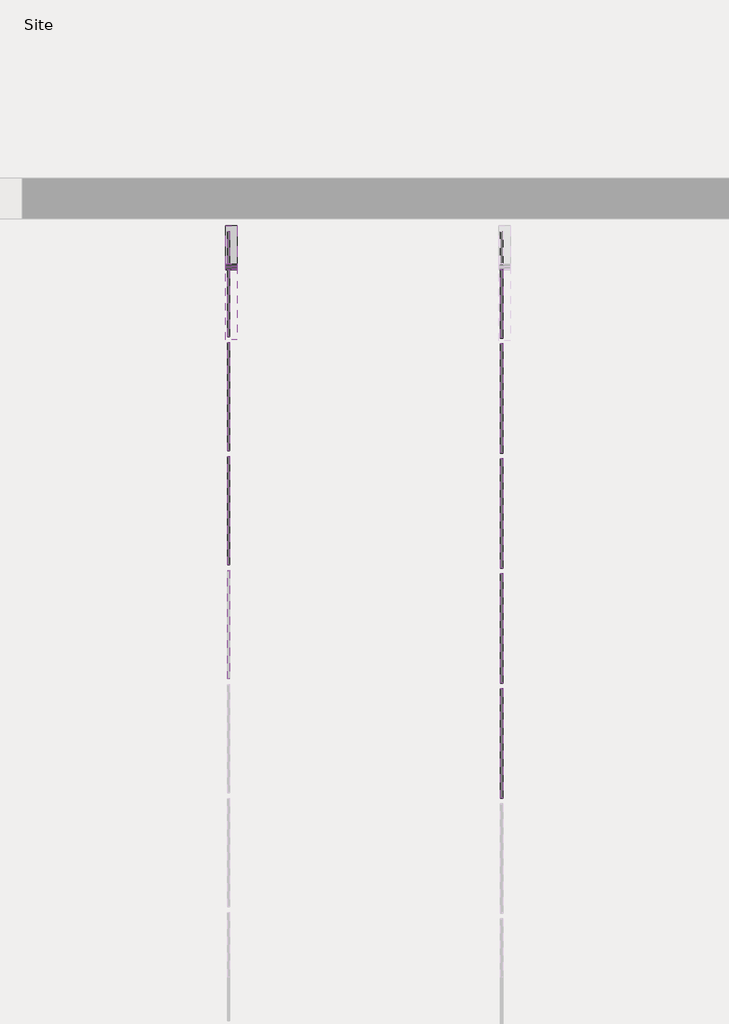
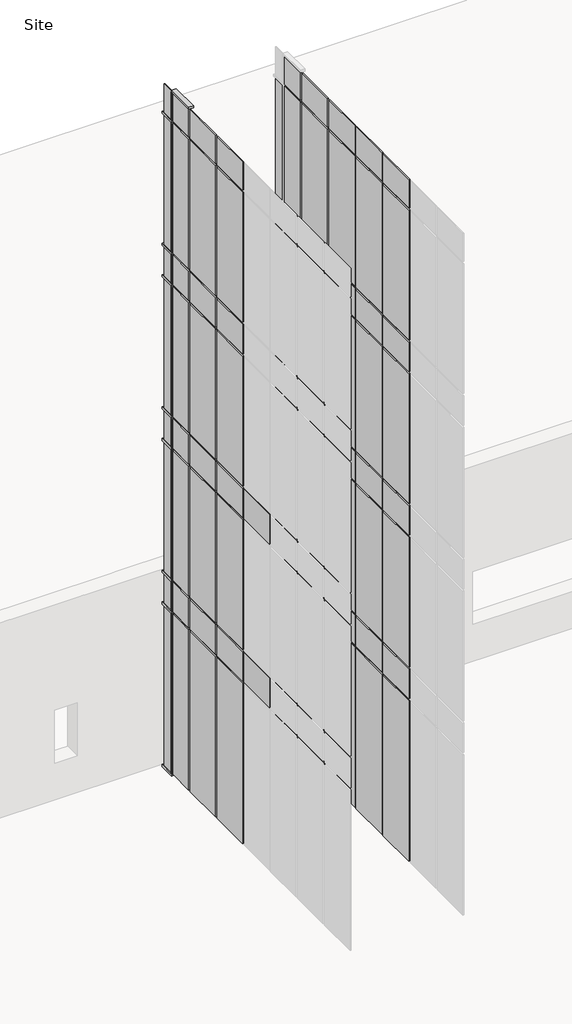
# One storey, part 3 of 4: 81 plates, 17 members.
"""IFC4 building model written with IfcOpenShell, lengths in millimetres."""

import ifcopenshell
import ifcopenshell.guid

model = None  # the IFC model being written
_history = None  # IfcOwnerHistory: only IFC2X3 demands one
_inside = {}  # id of a spatial element -> (the spatial element, [elements in it])
_under = {}  # id of a project, library or spatial element -> (it, [spatial elements below it])
_declared = {}  # id of a project -> (the project, [libraries it declares])
_typed = {}  # id of a type object -> (the type object, [elements of that type])
_made_of = {}  # id of a material, layer set ... -> (it, [elements and type objects made of it])


def new_model(schema):
    """Start an empty IFC model of exactly this schema.

    Asked for "IFC4X3", IfcOpenShell would pick the latest addendum, in which some entities
    have other attributes; the version numbers below select the first issue.
    IFC2X3 requires an IfcOwnerHistory on every rooted entity: one is made here for all.
    """
    global model, _history
    if schema == "IFC4X3":
        model = ifcopenshell.file(schema_version=(4, 3, 0, 0))
    else:
        model = ifcopenshell.file(schema=schema)
    _inside.clear()
    _under.clear()
    _declared.clear()
    _typed.clear()
    _made_of.clear()
    _history = None
    if model.schema == "IFC2X3":
        org = make("IfcOrganization", Name="unknown")
        user = make(
            "IfcPersonAndOrganization",
            ThePerson=make("IfcPerson", FamilyName="unknown"),
            TheOrganization=org,
        )
        app = make(
            "IfcApplication",
            ApplicationDeveloper=org,
            Version="unknown",
            ApplicationFullName="unknown",
            ApplicationIdentifier="unknown",
        )
        _history = make(
            "IfcOwnerHistory",
            OwningUser=user,
            OwningApplication=app,
            ChangeAction="ADDED",
            CreationDate=0,
        )
    return model


def make(cls, **values):
    """One entity of the class cls with the attributes given. An attribute that is None is left unset."""
    return model.create_entity(
        cls, **{name: value for name, value in values.items() if value is not None}
    )


def rooted(cls, **values):
    """An entity with a GlobalId (a new one), such as an element, a storey or a relation."""
    return make(cls, GlobalId=ifcopenshell.guid.new(), OwnerHistory=_history, **values)


def si_unit(unit_type, name, prefix=None):
    """IfcSIUnit, for example si_unit("LENGTHUNIT", "METRE", prefix="MILLI")."""
    return make("IfcSIUnit", UnitType=unit_type, Prefix=prefix, Name=name)


def assignment(units):
    """IfcUnitAssignment: the units of a project."""
    return None if units is None else make("IfcUnitAssignment", Units=units)


def point(xyz):
    """IfcCartesianPoint."""
    return None if xyz is None else make("IfcCartesianPoint", Coordinates=xyz)


def direction(xyz):
    """IfcDirection."""
    return None if xyz is None else make("IfcDirection", DirectionRatios=xyz)


def frame(location, z_axis=None, x_axis=None):
    """IfcAxis2Placement3D, a coordinate frame: its origin and axes. An axis left out is left unset."""
    return make(
        "IfcAxis2Placement3D",
        Location=point(location),
        Axis=direction(z_axis),
        RefDirection=direction(x_axis),
    )


def origin():
    """The frame at (0, 0, 0) with its axes left unset."""
    return frame((0.0, 0.0, 0.0))


def origin_with_axes():
    """The frame at (0, 0, 0) with the z axis (0, 0, 1) and the x axis (1, 0, 0) written out."""
    return frame((0.0, 0.0, 0.0), z_axis=(0.0, 0.0, 1.0), x_axis=(1.0, 0.0, 0.0))


def place(relative_to, where):
    """IfcLocalPlacement: puts the frame where relative to a parent placement (None: the world)."""
    return make(
        "IfcLocalPlacement", PlacementRelTo=relative_to, RelativePlacement=where
    )


def context(
    kind, dimensions, precision=None, world=None, true_north=None, identifier=None
):
    """IfcGeometricRepresentationContext, for example the 3D "Model" context."""
    return make(
        "IfcGeometricRepresentationContext",
        ContextIdentifier=identifier,
        ContextType=kind,
        CoordinateSpaceDimension=dimensions,
        Precision=precision,
        WorldCoordinateSystem=world,
        TrueNorth=true_north,
    )


def project(units=None, contexts=None):
    """IfcProject with its units and contexts."""
    return rooted(
        "IfcProject",
        Name="project",
        RepresentationContexts=contexts,
        UnitsInContext=assignment(units),
    )


def spatial(cls, under=None, at=None, **own):
    """A site, building, storey or space (cls), placed at a placement, below another one or the project."""
    s = rooted(cls, ObjectPlacement=at, **own)
    if under is not None:
        _under.setdefault(under.id(), (under, []))[1].append(s)
    return s


def polyline(points):
    """IfcPolyline through the points."""
    return make("IfcPolyline", Points=[point(p) for p in points])


def outline(outer, holes=None, kind="AREA"):
    """IfcArbitraryClosedProfileDef: a profile drawn as a closed curve; with holes, ...WithVoids."""
    if holes is None:
        return make("IfcArbitraryClosedProfileDef", ProfileType=kind, OuterCurve=outer)
    return make(
        "IfcArbitraryProfileDefWithVoids",
        ProfileType=kind,
        OuterCurve=outer,
        InnerCurves=holes,
    )


def extrude(swept, where, along, depth):
    """IfcExtrudedAreaSolid: the profile swept, set in the frame where, extruded along a direction by depth."""
    return make(
        "IfcExtrudedAreaSolid",
        SweptArea=swept,
        Position=where,
        ExtrudedDirection=direction(along),
        Depth=depth,
    )


def shape(context_of_items, identifier, shape_type, items):
    """IfcShapeRepresentation: the items that make up one representation, for example the "Body"."""
    return make(
        "IfcShapeRepresentation",
        ContextOfItems=context_of_items,
        RepresentationIdentifier=identifier,
        RepresentationType=shape_type,
        Items=items,
    )


def source(mapping_origin, context_of_items, identifier, shape_type, items):
    """IfcRepresentationMap: a shape defined once, which mapped items show again and again."""
    return make(
        "IfcRepresentationMap",
        MappingOrigin=mapping_origin,
        MappedRepresentation=shape(context_of_items, identifier, shape_type, items),
    )


def transform(
    local_origin,
    x_axis=None,
    y_axis=None,
    z_axis=None,
    scale=None,
    scale2=None,
    scale3=None,
    uniform=True,
):
    """IfcCartesianTransformationOperator3D, or its non-uniform kind. x_axis, y_axis, z_axis: its Axis1, 2, 3."""
    if uniform:
        return make(
            "IfcCartesianTransformationOperator3D",
            Axis1=direction(x_axis),
            Axis2=direction(y_axis),
            LocalOrigin=point(local_origin),
            Scale=scale,
            Axis3=direction(z_axis),
        )
    return make(
        "IfcCartesianTransformationOperator3DnonUniform",
        Axis1=direction(x_axis),
        Axis2=direction(y_axis),
        LocalOrigin=point(local_origin),
        Scale=scale,
        Axis3=direction(z_axis),
        Scale2=scale2,
        Scale3=scale3,
    )


def mapped(mapping_source, mapping_target):
    """IfcMappedItem: shows the shape of a source again, moved by a transform."""
    return make(
        "IfcMappedItem", MappingSource=mapping_source, MappingTarget=mapping_target
    )


def made_of(thing, what):
    """Note that an element or type object is made of a material, layer set ...; save() writes the relation."""
    if what is not None:
        _made_of.setdefault(what.id(), (what, []))[1].append(thing)
    return thing


def element(
    cls,
    number,
    at=None,
    inside=None,
    cuts=None,
    type_object=None,
    material=None,
    context=None,
    identifier="Body",
    shape_type=None,
    held_by="IfcProductDefinitionShape",
    body=None,
    shapes=None,
    **own,
):
    """One element of the class cls, such as IfcWall. Its Tag is "e" and its number.

    at: its placement. inside: the storey or other place that contains it. cuts: it is an
    opening in that element (IfcRelVoidsElement). A single representation is given by context,
    identifier, shape_type and body (its items); several are given by shapes. held_by: the class
    of the entity that holds the representations. save() writes the other relations.
    """
    e = rooted(cls, Tag="e%d" % number, ObjectPlacement=at, **own)
    if body is not None:
        shapes = [shape(context, identifier, shape_type, body)]
    if shapes is not None:
        e.Representation = make(held_by, Representations=shapes)
    if inside is not None:
        _inside.setdefault(inside.id(), (inside, []))[1].append(e)
    if cuts is not None:
        rooted(
            "IfcRelVoidsElement", RelatingBuildingElement=cuts, RelatedOpeningElement=e
        )
    if type_object is not None:
        _typed.setdefault(type_object.id(), (type_object, []))[1].append(e)
    return made_of(e, material)


def aggregate(whole, parts):
    """IfcRelAggregates: a whole, such as a stair, and the parts it consists of."""
    return rooted("IfcRelAggregates", RelatingObject=whole, RelatedObjects=parts)


def save(model, path):
    """Write the relations noted so far, then the file.

    IfcRelAggregates (storeys below a building ...), IfcRelContainedInSpatialStructure (elements
    in a storey), IfcRelDefinesByType, IfcRelAssociatesMaterial and IfcRelDeclares: one each for
    every whole, place, type object, material and project.
    """
    for whole, parts in _under.values():
        aggregate(whole, parts)
    for where, things in _inside.values():
        rooted(
            "IfcRelContainedInSpatialStructure",
            RelatedElements=things,
            RelatingStructure=where,
        )
    for kind, things in _typed.values():
        rooted("IfcRelDefinesByType", RelatedObjects=things, RelatingType=kind)
    for what, things in _made_of.values():
        rooted("IfcRelAssociatesMaterial", RelatedObjects=things, RelatingMaterial=what)
    for by, libraries in _declared.values():
        rooted("IfcRelDeclares", RelatingContext=by, RelatedDefinitions=libraries)
    model.write(path)


def member_5d07894b(model_context):
    return source(origin(), model_context, "Body", "SweptSolid", [
        extrude(outline(polyline([(31.75, 63.5), (31.75, -63.5), (-31.75, -63.5), (-31.75, 63.5), (31.75, 63.5)])), frame((0.0, 0.0, -4629.15), z_axis=(0.0, 0.0, 1.0), x_axis=(1.0, 0.0, 0.0)), (0.0, 0.0, 1.0), 4629.15),
    ])


def member_3ba9e939(model_context):
    return source(origin(), model_context, "Body", "SweptSolid", [
        extrude(outline(polyline([(31.75, 63.5), (31.75, -63.5), (-31.75, -63.5), (-31.75, 63.5), (31.75, 63.5)])), frame((0.0, 0.0, -3746.5), z_axis=(0.0, 0.0, 1.0), x_axis=(1.0, 0.0, 0.0)), (0.0, 0.0, 1.0), 3746.5),
    ])


def member_ad567e07(model_context):
    return source(origin(), model_context, "Body", "SweptSolid", [
        extrude(outline(polyline([(31.75, 63.5), (31.75, -63.5), (-31.75, -63.5), (-31.75, 63.5), (31.75, 63.5)])), frame((0.0, 0.0, -819.15), z_axis=(0.0, 0.0, 1.0), x_axis=(1.0, 0.0, 0.0)), (0.0, 0.0, 1.0), 819.15),
    ])


def member_7db1855a(model_context):
    return source(origin(), model_context, "Body", "SweptSolid", [
        extrude(outline(polyline([(31.75, 63.5), (31.75, -63.5), (-31.75, -63.5), (-31.75, 63.5), (31.75, 63.5)])), frame((0.0, 0.0, -850.9), z_axis=(0.0, 0.0, 1.0), x_axis=(1.0, 0.0, 0.0)), (0.0, 0.0, 1.0), 850.9),
    ])


def member_7227ddca(model_context):
    return source(origin(), model_context, "Body", "SweptSolid", [
        extrude(outline(polyline([(0.0, 63.5), (0.0, -63.5), (-63.5, -63.5), (-63.5, 63.5), (0.0, 63.5)])), frame((0.0, 0.0, -813.7989637), z_axis=(0.0, 0.0, 1.0), x_axis=(1.0, 0.0, 0.0)), (0.0, 0.0, 1.0), 813.7989637),
    ])


def member_ffd4c858(model_context):
    return source(origin(), model_context, "Body", "SweptSolid", [
        extrude(outline(polyline([(31.75, 63.5), (31.75, -63.5), (-31.75, -63.5), (-31.75, 63.5), (31.75, 63.5)])), frame((0.0, 0.0, -457.2), z_axis=(0.0, 0.0, 1.0), x_axis=(1.0, 0.0, 0.0)), (0.0, 0.0, 1.0), 457.2),
    ])


def member_15823cb3(model_context):
    return source(origin(), model_context, "Body", "SweptSolid", [
        extrude(outline(polyline([(0.0, 63.5), (0.0, -63.5), (-63.5, -63.5), (-63.5, 63.5), (0.0, 63.5)])), frame((0.0, 0.0, -457.2), z_axis=(0.0, 0.0, 1.0), x_axis=(1.0, 0.0, 0.0)), (0.0, 0.0, 1.0), 457.2),
    ])


def system_panel_glazed_26f8e022(model_context):
    return source(origin(), model_context, "Body", "SweptSolid", [
        extrude(outline(polyline([(603.7494819, 19.05), (-603.7494819, 19.05), (-603.7494819, 44.45), (603.7494819, 44.45), (603.7494819, 19.05)])), origin_with_axes(), (0.0, 0.0, 1.0), 4629.15),
    ])


def system_panel_glazed_31d10065(model_context):
    return source(origin(), model_context, "Body", "SweptSolid", [
        extrude(outline(polyline([(609.6, 19.05), (-609.6, 19.05), (-609.6, 44.45), (609.6, 44.45), (609.6, 19.05)])), origin_with_axes(), (0.0, 0.0, 1.0), 4629.15),
    ])


def system_panel_glazed_ccbaed92(model_context):
    return source(origin(), model_context, "Body", "SweptSolid", [
        extrude(outline(polyline([(375.1494819, 19.05), (-375.1494819, 19.05), (-375.1494819, 44.45), (375.1494819, 44.45), (375.1494819, 19.05)])), origin_with_axes(), (0.0, 0.0, 1.0), 4629.15),
    ])


def system_panel_glazed_7dca4fa5(model_context):
    return source(origin(), model_context, "Body", "SweptSolid", [
        extrude(outline(polyline([(381.0, 19.05), (-381.0, 19.05), (-381.0, 44.45), (381.0, 44.45), (381.0, 19.05)])), origin_with_axes(), (0.0, 0.0, 1.0), 4629.15),
    ])


def system_panel_glazed_2b3d2baa(model_context):
    return source(origin(), model_context, "Body", "SweptSolid", [
        extrude(outline(polyline([(609.6, 19.05), (-609.6, 19.05), (-609.6, 44.45), (609.6, 44.45), (609.6, 19.05)])), origin_with_axes(), (0.0, 0.0, 1.0), 3746.5),
    ])


def system_panel_glazed_7e289b92(model_context):
    return source(origin(), model_context, "Body", "SweptSolid", [
        extrude(outline(polyline([(381.0, 19.05), (-381.0, 19.05), (-381.0, 44.45), (381.0, 44.45), (381.0, 19.05)])), origin_with_axes(), (0.0, 0.0, 1.0), 3746.5),
    ])


def system_panel_glazed_8fe7ab7d(model_context):
    return source(origin(), model_context, "Body", "SweptSolid", [
        extrude(outline(polyline([(609.6, 19.05), (-609.6, 19.05), (-609.6, 44.45), (609.6, 44.45), (609.6, 19.05)])), origin_with_axes(), (0.0, 0.0, 1.0), 850.9),
    ])


def system_panel_glazed_4fa5cbd7(model_context):
    return source(origin(), model_context, "Body", "SweptSolid", [
        extrude(outline(polyline([(381.0, 19.05), (-381.0, 19.05), (-381.0, 44.45), (381.0, 44.45), (381.0, 19.05)])), origin_with_axes(), (0.0, 0.0, 1.0), 850.9),
    ])


def system_panel_glazed_636dec6d(model_context):
    return source(origin(), model_context, "Body", "SweptSolid", [
        extrude(outline(polyline([(609.6, 19.05), (-609.6, 19.05), (-609.6, 44.45), (609.6, 44.45), (609.6, 19.05)])), origin_with_axes(), (0.0, 0.0, 1.0), 819.15),
    ])


def system_panel_glazed_99ba6c15(model_context):
    return source(origin(), model_context, "Body", "SweptSolid", [
        extrude(outline(polyline([(381.0, 19.05), (-381.0, 19.05), (-381.0, 44.45), (381.0, 44.45), (381.0, 19.05)])), origin_with_axes(), (0.0, 0.0, 1.0), 819.15),
    ])


def system_panel_glazed_35bb093a(model_context):
    return source(origin(), model_context, "Body", "SweptSolid", [
        extrude(outline(polyline([(603.7494819, 19.05), (-603.7494819, 19.05), (-603.7494819, 44.45), (603.7494819, 44.45), (603.7494819, 19.05)])), origin_with_axes(), (0.0, 0.0, 1.0), 3746.5),
    ])


def system_panel_glazed_f4d1d7f7(model_context):
    return source(origin(), model_context, "Body", "SweptSolid", [
        extrude(outline(polyline([(375.1494819, 19.05), (-375.1494819, 19.05), (-375.1494819, 44.45), (375.1494819, 44.45), (375.1494819, 19.05)])), origin_with_axes(), (0.0, 0.0, 1.0), 3746.5),
    ])


def system_panel_glazed_6e853645(model_context):
    return source(origin(), model_context, "Body", "SweptSolid", [
        extrude(outline(polyline([(180.975, 19.05), (-180.975, 19.05), (-180.975, 44.45), (180.975, 44.45), (180.975, 19.05)])), origin_with_axes(), (0.0, 0.0, 1.0), 4629.15),
    ])


def system_panel_glazed_5cc7900c(model_context):
    return source(origin(), model_context, "Body", "SweptSolid", [
        extrude(outline(polyline([(180.975, 19.05), (-180.975, 19.05), (-180.975, 44.45), (180.975, 44.45), (180.975, 19.05)])), origin_with_axes(), (0.0, 0.0, 1.0), 850.9),
    ])


def system_panel_glazed_032e4dab(model_context):
    return source(origin(), model_context, "Body", "SweptSolid", [
        extrude(outline(polyline([(180.975, 19.05), (-180.975, 19.05), (-180.975, 44.45), (180.975, 44.45), (180.975, 19.05)])), origin_with_axes(), (0.0, 0.0, 1.0), 3746.5),
    ])


def system_panel_metal_panel_947f48db(model_context):
    return source(origin(), model_context, "Body", "SweptSolid", [
        extrude(outline(polyline([(603.7494819, 19.05), (-603.7494819, 19.05), (-603.7494819, 44.45), (603.7494819, 44.45), (603.7494819, 19.05)])), origin_with_axes(), (0.0, 0.0, 1.0), 819.15),
    ])


def system_panel_metal_panel_e2dbf0ce(model_context):
    return source(origin(), model_context, "Body", "SweptSolid", [
        extrude(outline(polyline([(375.1494819, 19.05), (-375.1494819, 19.05), (-375.1494819, 44.45), (375.1494819, 44.45), (375.1494819, 19.05)])), origin_with_axes(), (0.0, 0.0, 1.0), 819.15),
    ])


def system_panel_metal_panel_dcd9a435(model_context):
    return source(origin(), model_context, "Body", "SweptSolid", [
        extrude(outline(polyline([(603.7494819, 19.05), (-603.7494819, 19.05), (-603.7494819, 44.45), (603.7494819, 44.45), (603.7494819, 19.05)])), origin_with_axes(), (0.0, 0.0, 1.0), 850.9),
    ])


def system_panel_metal_panel_ab4ce9b6(model_context):
    return source(origin(), model_context, "Body", "SweptSolid", [
        extrude(outline(polyline([(375.1494819, 19.05), (-375.1494819, 19.05), (-375.1494819, 44.45), (375.1494819, 44.45), (375.1494819, 19.05)])), origin_with_axes(), (0.0, 0.0, 1.0), 850.9),
    ])


def system_panel_glazed_cc98a0ec(model_context):
    return source(origin(), model_context, "Body", "SweptSolid", [
        extrude(outline(polyline([(180.975, 19.05), (-180.975, 19.05), (-180.975, 44.45), (180.975, 44.45), (180.975, 19.05)])), origin_with_axes(), (0.0, 0.0, 1.0), 819.15),
    ])


model = new_model("IFC4")

# Units and contexts
model_context = context("Model", 3, world=origin())
ifc_project = project(units=[si_unit("LENGTHUNIT", "METRE", prefix="MILLI")], contexts=[model_context])

# Site, building, storey
site = spatial("IfcSite", under=ifc_project)
building = spatial("IfcBuilding", under=site)
storey = spatial("IfcBuildingStorey", under=building, Name="Site", Elevation=-152.4)

# Members
placement = place(None, origin())
member_shape = member_5d07894b(model_context)
element("IfcMember", 1, ObjectType="Rectangular Mullion1 : 2.5\" x 5\" rectangular", at=placement, inside=storey, context=model_context, shape_type="MappedRepresentation", body=[
    mapped(member_shape, transform((7830.8276119, 37629.311889, -88.9), x_axis=(0.0, 1.0, 0.0), y_axis=(1.0, 0.0, 0.0), z_axis=(0.0, 0.0, -1.0))),
])
member_2_shape = member_3ba9e939(model_context)
element("IfcMember", 2, ObjectType="Rectangular Mullion1 : 2.5\" x 5\" rectangular", at=placement, inside=storey, context=model_context, shape_type="MappedRepresentation", body=[
    mapped(member_2_shape, transform((7830.8276119, 37629.311889, 14966.95), x_axis=(0.0, 1.0, 0.0), y_axis=(1.0, 0.0, 0.0), z_axis=(0.0, 0.0, -1.0))),
])
element("IfcMember", 3, ObjectType="Rectangular Mullion1 : 2.5\" x 5\" rectangular", at=placement, inside=storey, context=model_context, shape_type="MappedRepresentation", body=[
    mapped(member_2_shape, transform((7830.8276119, 37629.311889, 10242.55), x_axis=(0.0, 1.0, 0.0), y_axis=(1.0, 0.0, 0.0), z_axis=(0.0, 0.0, -1.0))),
])
element("IfcMember", 4, ObjectType="Rectangular Mullion1 : 2.5\" x 5\" rectangular", at=placement, inside=storey, context=model_context, shape_type="MappedRepresentation", body=[
    mapped(member_2_shape, transform((7830.8276119, 37629.311889, 5518.15), x_axis=(0.0, 1.0, 0.0), y_axis=(1.0, 0.0, 0.0), z_axis=(0.0, 0.0, -1.0))),
])
member_3_shape = member_ad567e07(model_context)
element("IfcMember", 5, ObjectType="Rectangular Mullion1 : 2.5\" x 5\" rectangular", at=placement, inside=storey, context=model_context, shape_type="MappedRepresentation", body=[
    mapped(member_3_shape, transform((7830.8276119, 37629.311889, 18776.95), x_axis=(0.0, 1.0, 0.0), y_axis=(1.0, 0.0, 0.0), z_axis=(0.0, 0.0, -1.0))),
])
member_4_shape = member_7db1855a(model_context)
element("IfcMember", 6, ObjectType="Rectangular Mullion1 : 2.5\" x 5\" rectangular", at=placement, inside=storey, context=model_context, shape_type="MappedRepresentation", body=[
    mapped(member_4_shape, transform((7830.8276119, 37629.311889, 4603.75), x_axis=(0.0, 1.0, 0.0), y_axis=(1.0, 0.0, 0.0), z_axis=(0.0, 0.0, -1.0))),
])
element("IfcMember", 7, ObjectType="Rectangular Mullion1 : 2.5\" x 5\" rectangular", at=placement, inside=storey, context=model_context, shape_type="MappedRepresentation", body=[
    mapped(member_4_shape, transform((7830.8276119, 37629.311889, 9328.15), x_axis=(0.0, 1.0, 0.0), y_axis=(1.0, 0.0, 0.0), z_axis=(0.0, 0.0, -1.0))),
])
element("IfcMember", 8, ObjectType="Rectangular Mullion1 : 2.5\" x 5\" rectangular", at=placement, inside=storey, context=model_context, shape_type="MappedRepresentation", body=[
    mapped(member_4_shape, transform((7830.8276119, 37629.311889, 14052.55), x_axis=(0.0, 1.0, 0.0), y_axis=(1.0, 0.0, 0.0), z_axis=(0.0, 0.0, -1.0))),
])
member_5_shape = member_7227ddca(model_context)
element("IfcMember", 9, ObjectType="Rectangular Mullion1 : 2.5\" x 5\" rectangular", at=placement, inside=storey, context=model_context, shape_type="MappedRepresentation", body=[
    mapped(member_5_shape, transform((7830.8276119, 37629.311889, 19659.6), x_axis=(0.0, 0.0, 1.0), y_axis=(1.0, 0.0, 0.0), z_axis=(0.0, 1.0, 0.0))),
])
member_6_shape = member_ffd4c858(model_context)
element("IfcMember", 10, ObjectType="Rectangular Mullion1 : 2.5\" x 5\" rectangular", at=placement, inside=storey, context=model_context, shape_type="MappedRepresentation", body=[
    mapped(member_6_shape, transform((7830.8276119, 38086.511889, 5486.4), x_axis=(0.0, 0.0, 1.0), y_axis=(1.0, 0.0, 0.0), z_axis=(0.0, 1.0, 0.0))),
])
element("IfcMember", 11, ObjectType="Rectangular Mullion1 : 2.5\" x 5\" rectangular", at=placement, inside=storey, context=model_context, shape_type="MappedRepresentation", body=[
    mapped(member_6_shape, transform((7830.8276119, 38086.511889, 10210.8), x_axis=(0.0, 0.0, 1.0), y_axis=(1.0, 0.0, 0.0), z_axis=(0.0, 1.0, 0.0))),
])
element("IfcMember", 12, ObjectType="Rectangular Mullion1 : 2.5\" x 5\" rectangular", at=placement, inside=storey, context=model_context, shape_type="MappedRepresentation", body=[
    mapped(member_6_shape, transform((7830.8276119, 38086.511889, 14935.2), x_axis=(0.0, 0.0, 1.0), y_axis=(1.0, 0.0, 0.0), z_axis=(0.0, 1.0, 0.0))),
])
element("IfcMember", 13, ObjectType="Rectangular Mullion1 : 2.5\" x 5\" rectangular", at=placement, inside=storey, context=model_context, shape_type="MappedRepresentation", body=[
    mapped(member_6_shape, transform((7830.8276119, 38086.511889, 18745.2), x_axis=(0.0, 0.0, 1.0), y_axis=(1.0, 0.0, 0.0), z_axis=(0.0, 1.0, 0.0))),
])
element("IfcMember", 14, ObjectType="Rectangular Mullion1 : 2.5\" x 5\" rectangular", at=placement, inside=storey, context=model_context, shape_type="MappedRepresentation", body=[
    mapped(member_6_shape, transform((7830.8276119, 38086.511889, 14020.8), x_axis=(0.0, 0.0, 1.0), y_axis=(1.0, 0.0, 0.0), z_axis=(0.0, 1.0, 0.0))),
])
element("IfcMember", 15, ObjectType="Rectangular Mullion1 : 2.5\" x 5\" rectangular", at=placement, inside=storey, context=model_context, shape_type="MappedRepresentation", body=[
    mapped(member_6_shape, transform((7830.8276119, 38086.511889, 9296.4), x_axis=(0.0, 0.0, 1.0), y_axis=(1.0, 0.0, 0.0), z_axis=(0.0, 1.0, 0.0))),
])
element("IfcMember", 16, ObjectType="Rectangular Mullion1 : 2.5\" x 5\" rectangular", at=placement, inside=storey, context=model_context, shape_type="MappedRepresentation", body=[
    mapped(member_6_shape, transform((7830.8276119, 38086.511889, 4572.0), x_axis=(0.0, 0.0, 1.0), y_axis=(1.0, 0.0, 0.0), z_axis=(0.0, 1.0, 0.0))),
])
member_7_shape = member_15823cb3(model_context)
element("IfcMember", 17, ObjectType="Rectangular Mullion1 : 2.5\" x 5\" rectangular", at=placement, inside=storey, context=model_context, shape_type="MappedRepresentation", body=[
    mapped(member_7_shape, transform((7830.8276119, 37629.311889, -152.4), x_axis=(0.0, 0.0, -1.0), y_axis=(1.0, 0.0, 0.0), z_axis=(0.0, -1.0, 0.0))),
])

# Plates
system_panel_glazed_shape = system_panel_glazed_26f8e022(model_context)
element("IfcPlate", 18, ObjectType="System Panel : Glazed", at=placement, inside=storey, context=model_context, shape_type="MappedRepresentation", body=[
    mapped(system_panel_glazed_shape, transform((7830.8276119, 36180.0134434, -88.9), x_axis=(0.0, 1.0, 0.0), y_axis=(-1.0, 0.0, 0.0), z_axis=(0.0, 0.0, 1.0))),
])
element("IfcPlate", 19, ObjectType="System Panel : Glazed", at=placement, inside=storey, context=model_context, shape_type="MappedRepresentation", body=[
    mapped(system_panel_glazed_shape, transform((7830.8276119, 34909.0144797, -88.9), x_axis=(0.0, 1.0, 0.0), y_axis=(-1.0, 0.0, 0.0), z_axis=(0.0, 0.0, 1.0))),
])
system_panel_glazed_2_shape = system_panel_glazed_31d10065(model_context)
element("IfcPlate", 20, ObjectType="System Panel : Glazed", at=placement, inside=storey, context=model_context, shape_type="MappedRepresentation", body=[
    mapped(system_panel_glazed_2_shape, transform((10878.8276119, 33597.061889, -88.9), x_axis=(0.0, 1.0, 0.0), y_axis=(-1.0, 0.0, 0.0), z_axis=(0.0, 0.0, 1.0))),
])
element("IfcPlate", 21, ObjectType="System Panel : Glazed", at=placement, inside=storey, context=model_context, shape_type="MappedRepresentation", body=[
    mapped(system_panel_glazed_2_shape, transform((10878.8276119, 36162.461889, -88.9), x_axis=(0.0, 1.0, 0.0), y_axis=(-1.0, 0.0, 0.0), z_axis=(0.0, 0.0, 1.0))),
])
element("IfcPlate", 22, ObjectType="System Panel : Glazed", at=placement, inside=storey, context=model_context, shape_type="MappedRepresentation", body=[
    mapped(system_panel_glazed_2_shape, transform((10878.8276119, 32314.361889, -88.9), x_axis=(0.0, 1.0, 0.0), y_axis=(-1.0, 0.0, 0.0), z_axis=(0.0, 0.0, 1.0))),
])
element("IfcPlate", 23, ObjectType="System Panel : Glazed", at=placement, inside=storey, context=model_context, shape_type="MappedRepresentation", body=[
    mapped(system_panel_glazed_2_shape, transform((10878.8276119, 34879.761889, -88.9), x_axis=(0.0, 1.0, 0.0), y_axis=(-1.0, 0.0, 0.0), z_axis=(0.0, 0.0, 1.0))),
])
system_panel_glazed_3_shape = system_panel_glazed_ccbaed92(model_context)
element("IfcPlate", 24, ObjectType="System Panel : Glazed", at=placement, inside=storey, context=model_context, shape_type="MappedRepresentation", body=[
    mapped(system_panel_glazed_3_shape, transform((7830.8276119, 37222.4124071, -88.9), x_axis=(0.0, 1.0, 0.0), y_axis=(-1.0, 0.0, 0.0), z_axis=(0.0, 0.0, 1.0))),
])
system_panel_glazed_4_shape = system_panel_glazed_7dca4fa5(model_context)
element("IfcPlate", 25, ObjectType="System Panel : Glazed", at=placement, inside=storey, context=model_context, shape_type="MappedRepresentation", body=[
    mapped(system_panel_glazed_4_shape, transform((10878.8276119, 37216.561889, -88.9), x_axis=(0.0, 1.0, 0.0), y_axis=(-1.0, 0.0, 0.0), z_axis=(0.0, 0.0, 1.0))),
])
system_panel_glazed_5_shape = system_panel_glazed_2b3d2baa(model_context)
element("IfcPlate", 26, ObjectType="System Panel : Glazed", at=placement, inside=storey, context=model_context, shape_type="MappedRepresentation", body=[
    mapped(system_panel_glazed_5_shape, transform((10878.8276119, 32314.361889, 14966.95), x_axis=(0.0, 1.0, 0.0), y_axis=(-1.0, 0.0, 0.0), z_axis=(0.0, 0.0, 1.0))),
])
element("IfcPlate", 27, ObjectType="System Panel : Glazed", at=placement, inside=storey, context=model_context, shape_type="MappedRepresentation", body=[
    mapped(system_panel_glazed_5_shape, transform((10878.8276119, 33597.061889, 14966.95), x_axis=(0.0, 1.0, 0.0), y_axis=(-1.0, 0.0, 0.0), z_axis=(0.0, 0.0, 1.0))),
])
element("IfcPlate", 28, ObjectType="System Panel : Glazed", at=placement, inside=storey, context=model_context, shape_type="MappedRepresentation", body=[
    mapped(system_panel_glazed_5_shape, transform((10878.8276119, 34879.761889, 14966.95), x_axis=(0.0, 1.0, 0.0), y_axis=(-1.0, 0.0, 0.0), z_axis=(0.0, 0.0, 1.0))),
])
element("IfcPlate", 29, ObjectType="System Panel : Glazed", at=placement, inside=storey, context=model_context, shape_type="MappedRepresentation", body=[
    mapped(system_panel_glazed_5_shape, transform((10878.8276119, 36162.461889, 14966.95), x_axis=(0.0, 1.0, 0.0), y_axis=(-1.0, 0.0, 0.0), z_axis=(0.0, 0.0, 1.0))),
])
element("IfcPlate", 30, ObjectType="System Panel : Glazed", at=placement, inside=storey, context=model_context, shape_type="MappedRepresentation", body=[
    mapped(system_panel_glazed_5_shape, transform((10878.8276119, 32314.361889, 10242.55), x_axis=(0.0, 1.0, 0.0), y_axis=(-1.0, 0.0, 0.0), z_axis=(0.0, 0.0, 1.0))),
])
element("IfcPlate", 31, ObjectType="System Panel : Glazed", at=placement, inside=storey, context=model_context, shape_type="MappedRepresentation", body=[
    mapped(system_panel_glazed_5_shape, transform((10878.8276119, 33597.061889, 10242.55), x_axis=(0.0, 1.0, 0.0), y_axis=(-1.0, 0.0, 0.0), z_axis=(0.0, 0.0, 1.0))),
])
element("IfcPlate", 32, ObjectType="System Panel : Glazed", at=placement, inside=storey, context=model_context, shape_type="MappedRepresentation", body=[
    mapped(system_panel_glazed_5_shape, transform((10878.8276119, 34879.761889, 10242.55), x_axis=(0.0, 1.0, 0.0), y_axis=(-1.0, 0.0, 0.0), z_axis=(0.0, 0.0, 1.0))),
])
element("IfcPlate", 33, ObjectType="System Panel : Glazed", at=placement, inside=storey, context=model_context, shape_type="MappedRepresentation", body=[
    mapped(system_panel_glazed_5_shape, transform((10878.8276119, 36162.461889, 10242.55), x_axis=(0.0, 1.0, 0.0), y_axis=(-1.0, 0.0, 0.0), z_axis=(0.0, 0.0, 1.0))),
])
element("IfcPlate", 34, ObjectType="System Panel : Glazed", at=placement, inside=storey, context=model_context, shape_type="MappedRepresentation", body=[
    mapped(system_panel_glazed_5_shape, transform((10878.8276119, 32314.361889, 5518.15), x_axis=(0.0, 1.0, 0.0), y_axis=(-1.0, 0.0, 0.0), z_axis=(0.0, 0.0, 1.0))),
])
element("IfcPlate", 35, ObjectType="System Panel : Glazed", at=placement, inside=storey, context=model_context, shape_type="MappedRepresentation", body=[
    mapped(system_panel_glazed_5_shape, transform((10878.8276119, 33597.061889, 5518.15), x_axis=(0.0, 1.0, 0.0), y_axis=(-1.0, 0.0, 0.0), z_axis=(0.0, 0.0, 1.0))),
])
element("IfcPlate", 36, ObjectType="System Panel : Glazed", at=placement, inside=storey, context=model_context, shape_type="MappedRepresentation", body=[
    mapped(system_panel_glazed_5_shape, transform((10878.8276119, 34879.761889, 5518.15), x_axis=(0.0, 1.0, 0.0), y_axis=(-1.0, 0.0, 0.0), z_axis=(0.0, 0.0, 1.0))),
])
element("IfcPlate", 37, ObjectType="System Panel : Glazed", at=placement, inside=storey, context=model_context, shape_type="MappedRepresentation", body=[
    mapped(system_panel_glazed_5_shape, transform((10878.8276119, 36162.461889, 5518.15), x_axis=(0.0, 1.0, 0.0), y_axis=(-1.0, 0.0, 0.0), z_axis=(0.0, 0.0, 1.0))),
])
system_panel_glazed_6_shape = system_panel_glazed_7e289b92(model_context)
element("IfcPlate", 38, ObjectType="System Panel : Glazed", at=placement, inside=storey, context=model_context, shape_type="MappedRepresentation", body=[
    mapped(system_panel_glazed_6_shape, transform((10878.8276119, 37216.561889, 14966.95), x_axis=(0.0, 1.0, 0.0), y_axis=(-1.0, 0.0, 0.0), z_axis=(0.0, 0.0, 1.0))),
])
element("IfcPlate", 39, ObjectType="System Panel : Glazed", at=placement, inside=storey, context=model_context, shape_type="MappedRepresentation", body=[
    mapped(system_panel_glazed_6_shape, transform((10878.8276119, 37216.561889, 10242.55), x_axis=(0.0, 1.0, 0.0), y_axis=(-1.0, 0.0, 0.0), z_axis=(0.0, 0.0, 1.0))),
])
element("IfcPlate", 40, ObjectType="System Panel : Glazed", at=placement, inside=storey, context=model_context, shape_type="MappedRepresentation", body=[
    mapped(system_panel_glazed_6_shape, transform((10878.8276119, 37216.561889, 5518.15), x_axis=(0.0, 1.0, 0.0), y_axis=(-1.0, 0.0, 0.0), z_axis=(0.0, 0.0, 1.0))),
])
system_panel_glazed_7_shape = system_panel_glazed_8fe7ab7d(model_context)
element("IfcPlate", 41, ObjectType="System Panel : Glazed", at=placement, inside=storey, context=model_context, shape_type="MappedRepresentation", body=[
    mapped(system_panel_glazed_7_shape, transform((10878.8276119, 32314.361889, 9328.15), x_axis=(0.0, 1.0, 0.0), y_axis=(-1.0, 0.0, 0.0), z_axis=(0.0, 0.0, 1.0))),
])
element("IfcPlate", 42, ObjectType="System Panel : Glazed", at=placement, inside=storey, context=model_context, shape_type="MappedRepresentation", body=[
    mapped(system_panel_glazed_7_shape, transform((10878.8276119, 33597.061889, 9328.15), x_axis=(0.0, 1.0, 0.0), y_axis=(-1.0, 0.0, 0.0), z_axis=(0.0, 0.0, 1.0))),
])
element("IfcPlate", 43, ObjectType="System Panel : Glazed", at=placement, inside=storey, context=model_context, shape_type="MappedRepresentation", body=[
    mapped(system_panel_glazed_7_shape, transform((10878.8276119, 34879.761889, 9328.15), x_axis=(0.0, 1.0, 0.0), y_axis=(-1.0, 0.0, 0.0), z_axis=(0.0, 0.0, 1.0))),
])
element("IfcPlate", 44, ObjectType="System Panel : Glazed", at=placement, inside=storey, context=model_context, shape_type="MappedRepresentation", body=[
    mapped(system_panel_glazed_7_shape, transform((10878.8276119, 36162.461889, 9328.15), x_axis=(0.0, 1.0, 0.0), y_axis=(-1.0, 0.0, 0.0), z_axis=(0.0, 0.0, 1.0))),
])
element("IfcPlate", 45, ObjectType="System Panel : Glazed", at=placement, inside=storey, context=model_context, shape_type="MappedRepresentation", body=[
    mapped(system_panel_glazed_7_shape, transform((10878.8276119, 32314.361889, 4603.75), x_axis=(0.0, 1.0, 0.0), y_axis=(-1.0, 0.0, 0.0), z_axis=(0.0, 0.0, 1.0))),
])
element("IfcPlate", 46, ObjectType="System Panel : Glazed", at=placement, inside=storey, context=model_context, shape_type="MappedRepresentation", body=[
    mapped(system_panel_glazed_7_shape, transform((10878.8276119, 33597.061889, 4603.75), x_axis=(0.0, 1.0, 0.0), y_axis=(-1.0, 0.0, 0.0), z_axis=(0.0, 0.0, 1.0))),
])
element("IfcPlate", 47, ObjectType="System Panel : Glazed", at=placement, inside=storey, context=model_context, shape_type="MappedRepresentation", body=[
    mapped(system_panel_glazed_7_shape, transform((10878.8276119, 34879.761889, 4603.75), x_axis=(0.0, 1.0, 0.0), y_axis=(-1.0, 0.0, 0.0), z_axis=(0.0, 0.0, 1.0))),
])
element("IfcPlate", 48, ObjectType="System Panel : Glazed", at=placement, inside=storey, context=model_context, shape_type="MappedRepresentation", body=[
    mapped(system_panel_glazed_7_shape, transform((10878.8276119, 36162.461889, 4603.75), x_axis=(0.0, 1.0, 0.0), y_axis=(-1.0, 0.0, 0.0), z_axis=(0.0, 0.0, 1.0))),
])
element("IfcPlate", 49, ObjectType="System Panel : Glazed", at=placement, inside=storey, context=model_context, shape_type="MappedRepresentation", body=[
    mapped(system_panel_glazed_7_shape, transform((10878.8276119, 32314.361889, 14052.55), x_axis=(0.0, 1.0, 0.0), y_axis=(-1.0, 0.0, 0.0), z_axis=(0.0, 0.0, 1.0))),
])
element("IfcPlate", 50, ObjectType="System Panel : Glazed", at=placement, inside=storey, context=model_context, shape_type="MappedRepresentation", body=[
    mapped(system_panel_glazed_7_shape, transform((10878.8276119, 33597.061889, 14052.55), x_axis=(0.0, 1.0, 0.0), y_axis=(-1.0, 0.0, 0.0), z_axis=(0.0, 0.0, 1.0))),
])
element("IfcPlate", 51, ObjectType="System Panel : Glazed", at=placement, inside=storey, context=model_context, shape_type="MappedRepresentation", body=[
    mapped(system_panel_glazed_7_shape, transform((10878.8276119, 34879.761889, 14052.55), x_axis=(0.0, 1.0, 0.0), y_axis=(-1.0, 0.0, 0.0), z_axis=(0.0, 0.0, 1.0))),
])
element("IfcPlate", 52, ObjectType="System Panel : Glazed", at=placement, inside=storey, context=model_context, shape_type="MappedRepresentation", body=[
    mapped(system_panel_glazed_7_shape, transform((10878.8276119, 36162.461889, 14052.55), x_axis=(0.0, 1.0, 0.0), y_axis=(-1.0, 0.0, 0.0), z_axis=(0.0, 0.0, 1.0))),
])
system_panel_glazed_8_shape = system_panel_glazed_4fa5cbd7(model_context)
element("IfcPlate", 53, ObjectType="System Panel : Glazed", at=placement, inside=storey, context=model_context, shape_type="MappedRepresentation", body=[
    mapped(system_panel_glazed_8_shape, transform((10878.8276119, 37216.561889, 9328.15), x_axis=(0.0, 1.0, 0.0), y_axis=(-1.0, 0.0, 0.0), z_axis=(0.0, 0.0, 1.0))),
])
element("IfcPlate", 54, ObjectType="System Panel : Glazed", at=placement, inside=storey, context=model_context, shape_type="MappedRepresentation", body=[
    mapped(system_panel_glazed_8_shape, transform((10878.8276119, 37216.561889, 4603.75), x_axis=(0.0, 1.0, 0.0), y_axis=(-1.0, 0.0, 0.0), z_axis=(0.0, 0.0, 1.0))),
])
element("IfcPlate", 55, ObjectType="System Panel : Glazed", at=placement, inside=storey, context=model_context, shape_type="MappedRepresentation", body=[
    mapped(system_panel_glazed_8_shape, transform((10878.8276119, 37216.561889, 14052.55), x_axis=(0.0, 1.0, 0.0), y_axis=(-1.0, 0.0, 0.0), z_axis=(0.0, 0.0, 1.0))),
])
system_panel_glazed_9_shape = system_panel_glazed_636dec6d(model_context)
element("IfcPlate", 56, ObjectType="System Panel : Glazed", at=placement, inside=storey, context=model_context, shape_type="MappedRepresentation", body=[
    mapped(system_panel_glazed_9_shape, transform((10878.8276119, 32314.361889, 18776.95), x_axis=(0.0, 1.0, 0.0), y_axis=(-1.0, 0.0, 0.0), z_axis=(0.0, 0.0, 1.0))),
])
element("IfcPlate", 57, ObjectType="System Panel : Glazed", at=placement, inside=storey, context=model_context, shape_type="MappedRepresentation", body=[
    mapped(system_panel_glazed_9_shape, transform((10878.8276119, 33597.061889, 18776.95), x_axis=(0.0, 1.0, 0.0), y_axis=(-1.0, 0.0, 0.0), z_axis=(0.0, 0.0, 1.0))),
])
element("IfcPlate", 58, ObjectType="System Panel : Glazed", at=placement, inside=storey, context=model_context, shape_type="MappedRepresentation", body=[
    mapped(system_panel_glazed_9_shape, transform((10878.8276119, 34879.761889, 18776.95), x_axis=(0.0, 1.0, 0.0), y_axis=(-1.0, 0.0, 0.0), z_axis=(0.0, 0.0, 1.0))),
])
element("IfcPlate", 59, ObjectType="System Panel : Glazed", at=placement, inside=storey, context=model_context, shape_type="MappedRepresentation", body=[
    mapped(system_panel_glazed_9_shape, transform((10878.8276119, 36162.461889, 18776.95), x_axis=(0.0, 1.0, 0.0), y_axis=(-1.0, 0.0, 0.0), z_axis=(0.0, 0.0, 1.0))),
])
system_panel_glazed_10_shape = system_panel_glazed_99ba6c15(model_context)
element("IfcPlate", 60, ObjectType="System Panel : Glazed", at=placement, inside=storey, context=model_context, shape_type="MappedRepresentation", body=[
    mapped(system_panel_glazed_10_shape, transform((10878.8276119, 37216.561889, 18776.95), x_axis=(0.0, 1.0, 0.0), y_axis=(-1.0, 0.0, 0.0), z_axis=(0.0, 0.0, 1.0))),
])
system_panel_glazed_11_shape = system_panel_glazed_35bb093a(model_context)
element("IfcPlate", 61, ObjectType="System Panel : Glazed", at=placement, inside=storey, context=model_context, shape_type="MappedRepresentation", body=[
    mapped(system_panel_glazed_11_shape, transform((7830.8276119, 34909.0144797, 5518.15), x_axis=(0.0, 1.0, 0.0), y_axis=(-1.0, 0.0, 0.0), z_axis=(0.0, 0.0, 1.0))),
])
element("IfcPlate", 62, ObjectType="System Panel : Glazed", at=placement, inside=storey, context=model_context, shape_type="MappedRepresentation", body=[
    mapped(system_panel_glazed_11_shape, transform((7830.8276119, 36180.0134434, 5518.15), x_axis=(0.0, 1.0, 0.0), y_axis=(-1.0, 0.0, 0.0), z_axis=(0.0, 0.0, 1.0))),
])
element("IfcPlate", 63, ObjectType="System Panel : Glazed", at=placement, inside=storey, context=model_context, shape_type="MappedRepresentation", body=[
    mapped(system_panel_glazed_11_shape, transform((7830.8276119, 34909.0144797, 10242.55), x_axis=(0.0, 1.0, 0.0), y_axis=(-1.0, 0.0, 0.0), z_axis=(0.0, 0.0, 1.0))),
])
element("IfcPlate", 64, ObjectType="System Panel : Glazed", at=placement, inside=storey, context=model_context, shape_type="MappedRepresentation", body=[
    mapped(system_panel_glazed_11_shape, transform((7830.8276119, 36180.0134434, 10242.55), x_axis=(0.0, 1.0, 0.0), y_axis=(-1.0, 0.0, 0.0), z_axis=(0.0, 0.0, 1.0))),
])
element("IfcPlate", 65, ObjectType="System Panel : Glazed", at=placement, inside=storey, context=model_context, shape_type="MappedRepresentation", body=[
    mapped(system_panel_glazed_11_shape, transform((7830.8276119, 34909.0144797, 14966.95), x_axis=(0.0, 1.0, 0.0), y_axis=(-1.0, 0.0, 0.0), z_axis=(0.0, 0.0, 1.0))),
])
element("IfcPlate", 66, ObjectType="System Panel : Glazed", at=placement, inside=storey, context=model_context, shape_type="MappedRepresentation", body=[
    mapped(system_panel_glazed_11_shape, transform((7830.8276119, 36180.0134434, 14966.95), x_axis=(0.0, 1.0, 0.0), y_axis=(-1.0, 0.0, 0.0), z_axis=(0.0, 0.0, 1.0))),
])
system_panel_glazed_12_shape = system_panel_glazed_f4d1d7f7(model_context)
element("IfcPlate", 67, ObjectType="System Panel : Glazed", at=placement, inside=storey, context=model_context, shape_type="MappedRepresentation", body=[
    mapped(system_panel_glazed_12_shape, transform((7830.8276119, 37222.4124071, 5518.15), x_axis=(0.0, 1.0, 0.0), y_axis=(-1.0, 0.0, 0.0), z_axis=(0.0, 0.0, 1.0))),
])
element("IfcPlate", 68, ObjectType="System Panel : Glazed", at=placement, inside=storey, context=model_context, shape_type="MappedRepresentation", body=[
    mapped(system_panel_glazed_12_shape, transform((7830.8276119, 37222.4124071, 10242.55), x_axis=(0.0, 1.0, 0.0), y_axis=(-1.0, 0.0, 0.0), z_axis=(0.0, 0.0, 1.0))),
])
element("IfcPlate", 69, ObjectType="System Panel : Glazed", at=placement, inside=storey, context=model_context, shape_type="MappedRepresentation", body=[
    mapped(system_panel_glazed_12_shape, transform((7830.8276119, 37222.4124071, 14966.95), x_axis=(0.0, 1.0, 0.0), y_axis=(-1.0, 0.0, 0.0), z_axis=(0.0, 0.0, 1.0))),
])
system_panel_glazed_13_shape = system_panel_glazed_6e853645(model_context)
element("IfcPlate", 70, ObjectType="System Panel : Glazed", at=placement, inside=storey, context=model_context, shape_type="MappedRepresentation", body=[
    mapped(system_panel_glazed_13_shape, transform((10878.8276119, 37842.036889, -88.9), x_axis=(0.0, 1.0, 0.0), y_axis=(-1.0, 0.0, 0.0), z_axis=(0.0, 0.0, 1.0))),
])
system_panel_glazed_14_shape = system_panel_glazed_5cc7900c(model_context)
element("IfcPlate", 71, ObjectType="System Panel : Glazed", at=placement, inside=storey, context=model_context, shape_type="MappedRepresentation", body=[
    mapped(system_panel_glazed_14_shape, transform((10878.8276119, 37842.036889, 4603.75), x_axis=(0.0, 1.0, 0.0), y_axis=(-1.0, 0.0, 0.0), z_axis=(0.0, 0.0, 1.0))),
])
element("IfcPlate", 72, ObjectType="System Panel : Glazed", at=placement, inside=storey, context=model_context, shape_type="MappedRepresentation", body=[
    mapped(system_panel_glazed_14_shape, transform((10878.8276119, 37842.036889, 9328.15), x_axis=(0.0, 1.0, 0.0), y_axis=(-1.0, 0.0, 0.0), z_axis=(0.0, 0.0, 1.0))),
])
element("IfcPlate", 73, ObjectType="System Panel : Glazed", at=placement, inside=storey, context=model_context, shape_type="MappedRepresentation", body=[
    mapped(system_panel_glazed_14_shape, transform((10878.8276119, 37842.036889, 14052.55), x_axis=(0.0, 1.0, 0.0), y_axis=(-1.0, 0.0, 0.0), z_axis=(0.0, 0.0, 1.0))),
])
system_panel_glazed_15_shape = system_panel_glazed_032e4dab(model_context)
element("IfcPlate", 74, ObjectType="System Panel : Glazed", at=placement, inside=storey, context=model_context, shape_type="MappedRepresentation", body=[
    mapped(system_panel_glazed_15_shape, transform((10878.8276119, 37842.036889, 5518.15), x_axis=(0.0, 1.0, 0.0), y_axis=(-1.0, 0.0, 0.0), z_axis=(0.0, 0.0, 1.0))),
])
element("IfcPlate", 75, ObjectType="System Panel : Glazed", at=placement, inside=storey, context=model_context, shape_type="MappedRepresentation", body=[
    mapped(system_panel_glazed_15_shape, transform((10878.8276119, 37842.036889, 10242.55), x_axis=(0.0, 1.0, 0.0), y_axis=(-1.0, 0.0, 0.0), z_axis=(0.0, 0.0, 1.0))),
])
element("IfcPlate", 76, ObjectType="System Panel : Glazed", at=placement, inside=storey, context=model_context, shape_type="MappedRepresentation", body=[
    mapped(system_panel_glazed_15_shape, transform((10878.8276119, 37842.036889, 14966.95), x_axis=(0.0, 1.0, 0.0), y_axis=(-1.0, 0.0, 0.0), z_axis=(0.0, 0.0, 1.0))),
])
system_panel_metal_panel_shape = system_panel_metal_panel_947f48db(model_context)
element("IfcPlate", 77, ObjectType="System Panel : Metal Panel", at=placement, inside=storey, context=model_context, shape_type="MappedRepresentation", body=[
    mapped(system_panel_metal_panel_shape, transform((7830.8276119, 34909.0144797, 18776.95), x_axis=(0.0, 1.0, 0.0), y_axis=(-1.0, 0.0, 0.0), z_axis=(0.0, 0.0, 1.0))),
])
element("IfcPlate", 78, ObjectType="System Panel : Metal Panel", at=placement, inside=storey, context=model_context, shape_type="MappedRepresentation", body=[
    mapped(system_panel_metal_panel_shape, transform((7830.8276119, 36180.0134434, 18776.95), x_axis=(0.0, 1.0, 0.0), y_axis=(-1.0, 0.0, 0.0), z_axis=(0.0, 0.0, 1.0))),
])
system_panel_metal_panel_2_shape = system_panel_metal_panel_e2dbf0ce(model_context)
element("IfcPlate", 79, ObjectType="System Panel : Metal Panel", at=placement, inside=storey, context=model_context, shape_type="MappedRepresentation", body=[
    mapped(system_panel_metal_panel_2_shape, transform((7830.8276119, 37222.4124071, 18776.95), x_axis=(0.0, 1.0, 0.0), y_axis=(-1.0, 0.0, 0.0), z_axis=(0.0, 0.0, 1.0))),
])
system_panel_metal_panel_3_shape = system_panel_metal_panel_dcd9a435(model_context)
element("IfcPlate", 80, ObjectType="System Panel : Metal Panel", at=placement, inside=storey, context=model_context, shape_type="MappedRepresentation", body=[
    mapped(system_panel_metal_panel_3_shape, transform((7830.8276119, 34909.0144797, 14052.55), x_axis=(0.0, 1.0, 0.0), y_axis=(-1.0, 0.0, 0.0), z_axis=(0.0, 0.0, 1.0))),
])
element("IfcPlate", 81, ObjectType="System Panel : Metal Panel", at=placement, inside=storey, context=model_context, shape_type="MappedRepresentation", body=[
    mapped(system_panel_metal_panel_3_shape, transform((7830.8276119, 36180.0134434, 14052.55), x_axis=(0.0, 1.0, 0.0), y_axis=(-1.0, 0.0, 0.0), z_axis=(0.0, 0.0, 1.0))),
])
element("IfcPlate", 82, ObjectType="System Panel : Metal Panel", at=placement, inside=storey, context=model_context, shape_type="MappedRepresentation", body=[
    mapped(system_panel_metal_panel_3_shape, transform((7830.8276119, 33638.015516, 9328.15), x_axis=(0.0, 1.0, 0.0), y_axis=(-1.0, 0.0, 0.0), z_axis=(0.0, 0.0, 1.0))),
])
element("IfcPlate", 83, ObjectType="System Panel : Metal Panel", at=placement, inside=storey, context=model_context, shape_type="MappedRepresentation", body=[
    mapped(system_panel_metal_panel_3_shape, transform((7830.8276119, 34909.0144797, 9328.15), x_axis=(0.0, 1.0, 0.0), y_axis=(-1.0, 0.0, 0.0), z_axis=(0.0, 0.0, 1.0))),
])
element("IfcPlate", 84, ObjectType="System Panel : Metal Panel", at=placement, inside=storey, context=model_context, shape_type="MappedRepresentation", body=[
    mapped(system_panel_metal_panel_3_shape, transform((7830.8276119, 36180.0134434, 9328.15), x_axis=(0.0, 1.0, 0.0), y_axis=(-1.0, 0.0, 0.0), z_axis=(0.0, 0.0, 1.0))),
])
element("IfcPlate", 85, ObjectType="System Panel : Metal Panel", at=placement, inside=storey, context=model_context, shape_type="MappedRepresentation", body=[
    mapped(system_panel_metal_panel_3_shape, transform((7830.8276119, 33638.015516, 4603.75), x_axis=(0.0, 1.0, 0.0), y_axis=(-1.0, 0.0, 0.0), z_axis=(0.0, 0.0, 1.0))),
])
element("IfcPlate", 86, ObjectType="System Panel : Metal Panel", at=placement, inside=storey, context=model_context, shape_type="MappedRepresentation", body=[
    mapped(system_panel_metal_panel_3_shape, transform((7830.8276119, 34909.0144797, 4603.75), x_axis=(0.0, 1.0, 0.0), y_axis=(-1.0, 0.0, 0.0), z_axis=(0.0, 0.0, 1.0))),
])
element("IfcPlate", 87, ObjectType="System Panel : Metal Panel", at=placement, inside=storey, context=model_context, shape_type="MappedRepresentation", body=[
    mapped(system_panel_metal_panel_3_shape, transform((7830.8276119, 36180.0134434, 4603.75), x_axis=(0.0, 1.0, 0.0), y_axis=(-1.0, 0.0, 0.0), z_axis=(0.0, 0.0, 1.0))),
])
system_panel_metal_panel_4_shape = system_panel_metal_panel_ab4ce9b6(model_context)
element("IfcPlate", 88, ObjectType="System Panel : Metal Panel", at=placement, inside=storey, context=model_context, shape_type="MappedRepresentation", body=[
    mapped(system_panel_metal_panel_4_shape, transform((7830.8276119, 37222.4124071, 14052.55), x_axis=(0.0, 1.0, 0.0), y_axis=(-1.0, 0.0, 0.0), z_axis=(0.0, 0.0, 1.0))),
])
element("IfcPlate", 89, ObjectType="System Panel : Metal Panel", at=placement, inside=storey, context=model_context, shape_type="MappedRepresentation", body=[
    mapped(system_panel_metal_panel_4_shape, transform((7830.8276119, 37222.4124071, 9328.15), x_axis=(0.0, 1.0, 0.0), y_axis=(-1.0, 0.0, 0.0), z_axis=(0.0, 0.0, 1.0))),
])
element("IfcPlate", 90, ObjectType="System Panel : Metal Panel", at=placement, inside=storey, context=model_context, shape_type="MappedRepresentation", body=[
    mapped(system_panel_metal_panel_4_shape, transform((7830.8276119, 37222.4124071, 4603.75), x_axis=(0.0, 1.0, 0.0), y_axis=(-1.0, 0.0, 0.0), z_axis=(0.0, 0.0, 1.0))),
])
element("IfcPlate", 91, ObjectType="System Panel : Metal Panel", at=placement, inside=storey, context=model_context, shape_type="MappedRepresentation", body=[
    mapped(system_panel_glazed_13_shape, transform((7830.8276119, 37842.036889, -88.9), x_axis=(0.0, 1.0, 0.0), y_axis=(-1.0, 0.0, 0.0), z_axis=(0.0, 0.0, 1.0))),
])
element("IfcPlate", 92, ObjectType="System Panel : Metal Panel", at=placement, inside=storey, context=model_context, shape_type="MappedRepresentation", body=[
    mapped(system_panel_glazed_14_shape, transform((7830.8276119, 37842.036889, 4603.75), x_axis=(0.0, 1.0, 0.0), y_axis=(-1.0, 0.0, 0.0), z_axis=(0.0, 0.0, 1.0))),
])
element("IfcPlate", 93, ObjectType="System Panel : Metal Panel", at=placement, inside=storey, context=model_context, shape_type="MappedRepresentation", body=[
    mapped(system_panel_glazed_14_shape, transform((7830.8276119, 37842.036889, 9328.15), x_axis=(0.0, 1.0, 0.0), y_axis=(-1.0, 0.0, 0.0), z_axis=(0.0, 0.0, 1.0))),
])
element("IfcPlate", 94, ObjectType="System Panel : Metal Panel", at=placement, inside=storey, context=model_context, shape_type="MappedRepresentation", body=[
    mapped(system_panel_glazed_14_shape, transform((7830.8276119, 37842.036889, 14052.55), x_axis=(0.0, 1.0, 0.0), y_axis=(-1.0, 0.0, 0.0), z_axis=(0.0, 0.0, 1.0))),
])
element("IfcPlate", 95, ObjectType="System Panel : Metal Panel", at=placement, inside=storey, context=model_context, shape_type="MappedRepresentation", body=[
    mapped(system_panel_glazed_15_shape, transform((7830.8276119, 37842.036889, 5518.15), x_axis=(0.0, 1.0, 0.0), y_axis=(-1.0, 0.0, 0.0), z_axis=(0.0, 0.0, 1.0))),
])
element("IfcPlate", 96, ObjectType="System Panel : Metal Panel", at=placement, inside=storey, context=model_context, shape_type="MappedRepresentation", body=[
    mapped(system_panel_glazed_15_shape, transform((7830.8276119, 37842.036889, 10242.55), x_axis=(0.0, 1.0, 0.0), y_axis=(-1.0, 0.0, 0.0), z_axis=(0.0, 0.0, 1.0))),
])
element("IfcPlate", 97, ObjectType="System Panel : Metal Panel", at=placement, inside=storey, context=model_context, shape_type="MappedRepresentation", body=[
    mapped(system_panel_glazed_15_shape, transform((7830.8276119, 37842.036889, 14966.95), x_axis=(0.0, 1.0, 0.0), y_axis=(-1.0, 0.0, 0.0), z_axis=(0.0, 0.0, 1.0))),
])
system_panel_glazed_16_shape = system_panel_glazed_cc98a0ec(model_context)
element("IfcPlate", 98, ObjectType="System Panel : Metal Panel", at=placement, inside=storey, context=model_context, shape_type="MappedRepresentation", body=[
    mapped(system_panel_glazed_16_shape, transform((7830.8276119, 37842.036889, 18776.95), x_axis=(0.0, 1.0, 0.0), y_axis=(-1.0, 0.0, 0.0), z_axis=(0.0, 0.0, 1.0))),
])

save(model, "model.ifc")

# Revit data of these elements
# Type "Rectangular Mullion1 : 2.5\" x 5\" rectangular"
#   built-in parameter 1007304 = 0.416667 (stored number, unit not read)
#   built-in parameter 1007301 = 0.104167 (stored number, unit not read)
#   built-in parameter 1007300 = 0.104167 (stored number, unit not read)
# Type "System Panel : Glazed"
#   Construction Type Id = "GSP4R"
#   Analytic Construction = "1/8 in Pilkington single glazing"
#   Visual Light Transmittance = 0.9
#   Solar Heat Gain Coefficient = 0.86
#   Heat Transfer Coefficient (U) = 1.18115 BTU/(h·ft²·°F)
#   Define Thermal Properties by = 1
# Elements 1, 2, 3, 4, 5, 6, 7, 8, 9, 10, 11, 12, 13, 14, 15, 16, 17 (IfcMember, "Rectangular Mullion1 : 2.5\" x 5\" rectangular")
#   Phase Created = New Construction
#   Materials on its faces: "support-frame"
# Elements 18, 19, 20, 21, 22, 23, 24, 25, 26, 27, 28, 29, 30, 31, 32, 33, 34, 35, 36, 37, 38, 39, 40, 41, 42, 43, 44, 45, 46, 47, 48, 49, 50, 51, 52, 53, 54, 55, 56, 57, 58, 59, 60, 61, 62, 63, 64, 65, 66, 67, 68, 69, 70, 71, 72, 73, 74, 75, 76 (IfcPlate, "System Panel : Glazed")
#   Phase Created = New Construction
#   Materials on its faces: "Glass"
# Elements 77, 78, 79, 80, 81, 82, 83, 84, 85, 86, 87, 88, 89, 90, 91, 92, 93, 94, 95, 96, 97, 98 (IfcPlate, "System Panel : Metal Panel")
#   Phase Created = New Construction
#   Materials on its faces: "Aluminum"
# Materials
#   "support-frame": class "Unassigned", colour RGB 233 233 233, transparency 0, Cost = 0
#   "Glass": class "Glass", colour RGB 0 128 192, transparency 0.75, Description = "Soda Lime Glass", Cost = 0
#   "Aluminum": class "Metal", colour RGB 247 247 247, transparency 0, Description = "Aluminum 6061", Cost = 0
